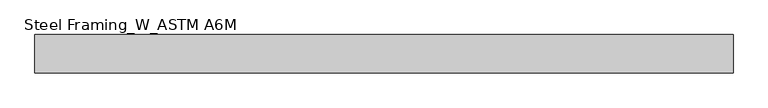
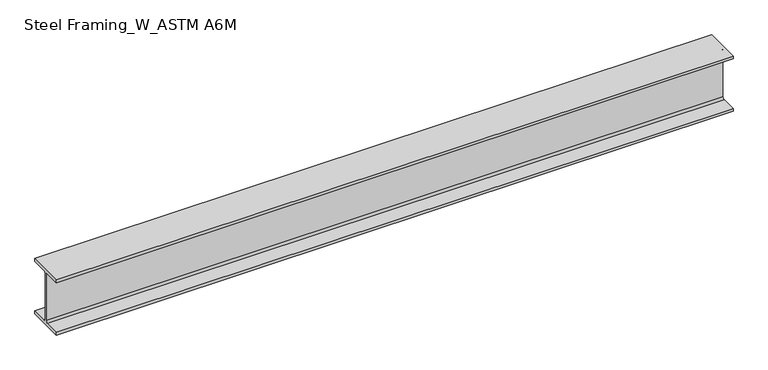
"""IFC4 building model written with IfcOpenShell, lengths in millimetres: beam geometry, Steel Framing_W_ASTM A6M : H_SB_AR_S02_W200x31.3_B6."""

from ifc_helpers import new_model, si_unit, point, frame, frame_2d, origin, place, context, project, spatial, polyline, circle_curve, trimmed, segment, composite_curve, outline, extrude, source, transform, mapped, element, save


def steel_framing_w_astm_a6m_5f04d38f(model_context):
    return source(origin(), model_context, "Body", "SweptSolid", [
        extrude(outline(composite_curve([segment(polyline([(67.0, -94.8), (67.0, -105.0), (-67.0, -105.0), (-67.0, -94.8), (-10.775, -94.8)]), True, "CONTINUOUS"), segment(trimmed(circle_curve(frame_2d((-10.775, -87.2)), 7.6), [point((-10.775, -94.8))], [point((-3.175, -87.2))], True, "CARTESIAN"), True, "CONTINUOUS"), segment(polyline([(-3.175, -87.2), (-3.175, 87.2)]), True, "CONTINUOUS"), segment(trimmed(circle_curve(frame_2d((-10.775, 87.2)), 7.6), [point((-3.175, 87.2))], [point((-10.775, 94.8))], True, "CARTESIAN"), True, "CONTINUOUS"), segment(polyline([(-10.775, 94.8), (-67.0, 94.8), (-67.0, 105.0), (67.0, 105.0), (67.0, 94.8), (10.775, 94.8)]), True, "CONTINUOUS"), segment(trimmed(circle_curve(frame_2d((10.775, 87.2)), 7.6), [point((10.775, 94.8))], [point((3.175, 87.2))], True, "CARTESIAN"), True, "CONTINUOUS"), segment(polyline([(3.175, 87.2), (3.175, -87.2)]), True, "CONTINUOUS"), segment(trimmed(circle_curve(frame_2d((10.775, -87.2)), 7.6), [point((3.175, -87.2))], [point((10.775, -94.8))], True, "CARTESIAN"), True, "CONTINUOUS"), segment(polyline([(10.775, -94.8), (67.0, -94.8)]), True, "CONTINUOUS")], self_intersect=False)), frame((-1181.3, 0.0, 0.0), z_axis=(1.0, 0.0, 0.0), x_axis=(0.0, 1.0, 0.0)), (0.0, 0.0, 1.0), 2436.6),
    ])


if __name__ == "__main__":
    model = new_model("IFC4")
    model_context = context("Model", 3, world=origin())
    ifc_project = project(units=[si_unit("LENGTHUNIT", "METRE", prefix="MILLI")], contexts=[model_context])
    site = spatial("IfcSite", under=ifc_project)
    building = spatial("IfcBuilding", under=site)
    placement = place(None, origin())
    steel_framing_w_astm_a6m_shape = steel_framing_w_astm_a6m_5f04d38f(model_context)
    element("IfcBeam", 1, ObjectType="Steel Framing_W_ASTM A6M : H_SB_AR_S02_W200x31.3_B6", at=placement, inside=building, context=model_context, shape_type="MappedRepresentation", body=[
        mapped(steel_framing_w_astm_a6m_shape, transform((0.0, 0.0, 0.0), x_axis=(1.0, 0.0, 0.0), y_axis=(0.0, 1.0, 0.0), z_axis=(0.0, 0.0, 1.0))),
    ])
    save(model, "model.ifc")

# Revit data of these elements
# Type "Steel Framing_W_ASTM A6M : H_SB_AR_S02_W200x31.3_B6"
#   Type Mark = "B6"
#   Section Name Key = "W8x21"
#   Width = 13.4 cm
#   Web Thickness = 0.635 cm
#   Web Fillet = 0.76 cm
#   Warping Constant = 40800.0 cm⁶
#   Torsional Moment of Inertia = 11.70 cm⁴
#   Section Area = 39.7 cm²
#   Plastic Modulus weak axis = 93.2 cm³
#   Plastic Modulus strong axis = 334.0 cm³
#   Perimeter = 0.93 m²/m
#   Nominal Weight = 31.30 kgf/m
#   Moment of Inertia weak axis = 407.00 cm⁴
#   Moment of Inertia strong axis = 3130.00 cm⁴
#   Height = 21.0 cm
#   Flange Thickness = 1.02 cm
#   Elastic Modulus weak axis = 60.8 cm³
#   Elastic Modulus strong axis = 298.0 cm³
#   Centroid Vertical = 10.5 cm
#   Centroid Horizontal = 6.7 cm
#   Length [instance default] = 1500 mm
#   Structural Material [instance default] = Steel, 45-345
#   Bolt Spacing = 0
#   Assembly Code = ""
# Element 1 (IfcBeam, "Steel Framing_W_ASTM A6M : H_SB_AR_S02_W200x31.3_B6")
#   Materials on its faces: "Steel, 45-345"
# Materials
#   "Steel, 45-345": class "Metal", colour RGB 189 187 185, transparency 0, Description = "Steel 345 MPa", Cost = 0
